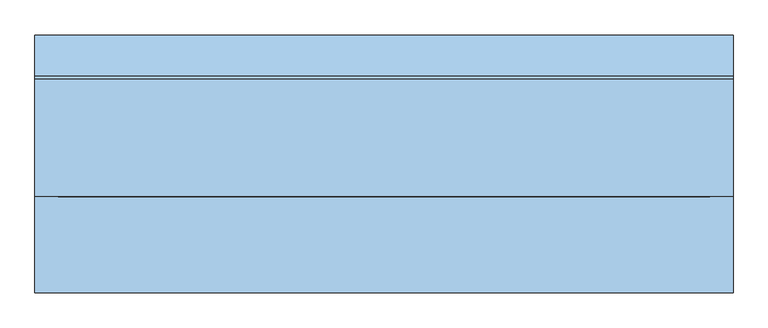
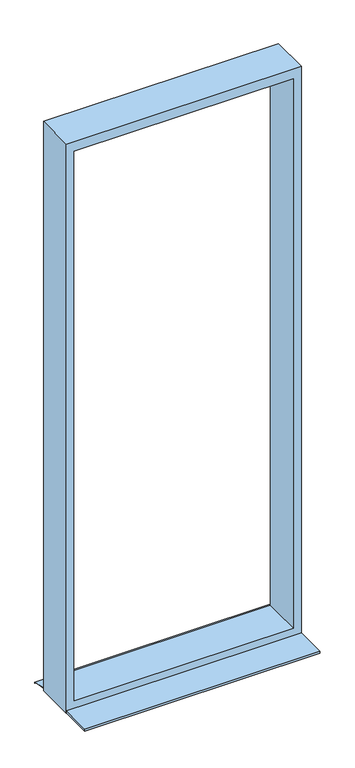
"""IFC4 building model written with IfcOpenShell, lengths in millimetres: window geometry, Fenster - Festverglasung : Feste Verglasung 4.58 x 1.79 3."""

from ifc_helpers import new_model, si_unit, frame, origin, place, context, project, spatial, polyline, outline, extrude, source, transform, mapped, element, save


def window_fd4d53b7(model_context):
    return source(origin(), model_context, "Body", "SweptSolid", [
        extrude(outline(polyline([(5580.0, 895.0), (5580.0, -895.0), (1000.0, -895.0), (1000.0, 895.0), (5580.0, 895.0)]), holes=[polyline([(5500.0, 835.0), (1080.0, 835.0), (1080.0, -835.0), (5500.0, -835.0), (5500.0, 835.0)])]), frame((0.0, -84.1317884, 0.0), z_axis=(0.0, 1.0, 0.0), x_axis=(0.0, 0.0, 1.0)), (0.0, 0.0, 1.0), 300.0),
        extrude(outline(polyline([(-895.0, -330.0), (-895.0, -84.1317884), (895.0, -84.1317884), (895.0, -330.0), (-895.0, -330.0)])), frame((0.0, 0.0, 1005.0), z_axis=(0.0, 0.0, 1.0), x_axis=(1.0, 0.0, 0.0)), (0.0, 0.0, 1.0), 15.0),
        extrude(outline(polyline([(225.8903659, 1020.0), (330.0, 1000.0), (330.0, 990.0), (328.0, 990.0), (328.0, 998.3604634), (225.6922839, 1018.0), (215.8682116, 1018.0), (215.8682116, 1020.0), (225.8903659, 1020.0)])), frame((-895.0, 0.0, 0.0), z_axis=(1.0, 0.0, 0.0), x_axis=(0.0, 1.0, 0.0)), (0.0, 0.0, 1.0), 1790.0),
    ])


if __name__ == "__main__":
    model = new_model("IFC4")
    model_context = context("Model", 3, world=origin())
    ifc_project = project(units=[si_unit("LENGTHUNIT", "METRE", prefix="MILLI")], contexts=[model_context])
    site = spatial("IfcSite", under=ifc_project)
    building = spatial("IfcBuilding", under=site)
    placement = place(None, origin())
    window_shape = window_fd4d53b7(model_context)
    element("IfcWindow", 1, ObjectType="Fenster - Festverglasung : Feste Verglasung 4.58 x 1.79 3", at=placement, inside=building, context=model_context, shape_type="MappedRepresentation", body=[
        mapped(window_shape, transform((0.0, 0.0, 0.0), x_axis=(1.0, 0.0, 0.0), y_axis=(0.0, 1.0, 0.0), z_axis=(0.0, 0.0, 1.0))),
    ])
    save(model, "model.ifc")

# Revit data of these elements
# Type "Fenster - Festverglasung : Feste Verglasung 4.58 x 1.79 3"
#   Type Mark = "61"
#   Operation = "SinglePanel"
#   Keynote = "16.05.01"
#   Visual Light Transmittance = 0.9
#   Solar Heat Gain Coefficient = 0.78
#   Rough Width = 1.790 m
#   Rough Height = 4.580 m
#   Heat Transfer Coefficient (U) = 3.6886 W/(m²·K)
#   Rahmentiefe = 0.300 m
#   Rahmenhöhe unten = 0.080 m
#   Höhe oberer  Rahmen = 0.080 m
#   Rahmenbreite = 0.060 m
#   Height = 4.580 m
#   Einbautiefe (von außen) [instance default] = 0.080 m
#   Width = 1.790 m
#   Wall Closure = 3
#   Bild [instance default] = none
#   Glas [instance default] = none
#   Innere Fensterbank [instance default] = none
#   Äußere Fensterbank [instance default] = none
#   Construction Type Id = ""
#   Analytic Construction = (empty or 0)
# Element 1 (IfcWindow, "Fenster - Festverglasung : Feste Verglasung 4.58 x 1.79 3")
#   Einbautiefe (von außen) = 0.084132 m
#   Materials on its faces: "Kunststoff - Weiß", "Holz - Birke"
# Materials
#   "Kunststoff - Weiß": class "Kunststoff", colour RGB 249 249 249, transparency 0, Cost = 0
#   "Holz - Birke": class "Holz", colour RGB 213 164 103, transparency 0, Cost = 0
